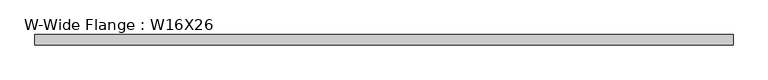
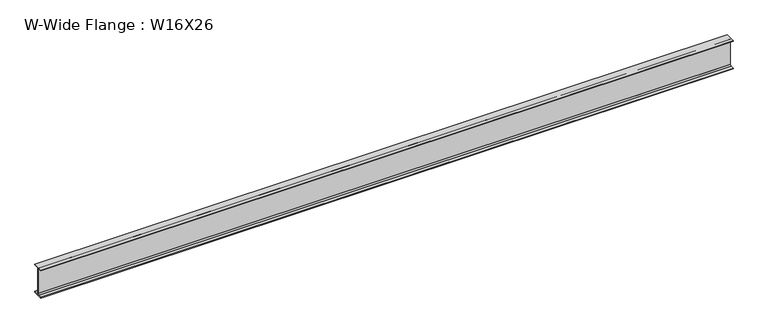
"""IFC4 building model written with IfcOpenShell, lengths in millimetres: beam geometry, W-Wide Flange : W16X26."""

from ifc_helpers import new_model, si_unit, point, frame, frame_2d, origin, place, context, project, spatial, polyline, circle_curve, trimmed, segment, composite_curve, outline, extrude, source, transform, mapped, element, save


def w_wide_flange_w16x26_70125ba5(model_context):
    return source(origin(), model_context, "Body", "SweptSolid", [
        extrude(outline(composite_curve([segment(polyline([(69.85, -190.627), (69.85, -199.39), (-69.85, -199.39), (-69.85, -190.627), (-21.3995, -190.627)]), True, "CONTINUOUS"), segment(trimmed(circle_curve(frame_2d((-21.3995, -172.4025)), 18.2245), [point((-21.3995, -190.627))], [point((-3.175, -172.4025))], True, "CARTESIAN"), True, "CONTINUOUS"), segment(polyline([(-3.175, -172.4025), (-3.175, 172.4025)]), True, "CONTINUOUS"), segment(trimmed(circle_curve(frame_2d((-21.3995, 172.4025)), 18.2245), [point((-3.175, 172.4025))], [point((-21.3995, 190.627))], True, "CARTESIAN"), True, "CONTINUOUS"), segment(polyline([(-21.3995, 190.627), (-69.85, 190.627), (-69.85, 199.39), (69.85, 199.39), (69.85, 190.627), (21.3995, 190.627)]), True, "CONTINUOUS"), segment(trimmed(circle_curve(frame_2d((21.3995, 172.4025)), 18.2245), [point((21.3995, 190.627))], [point((3.175, 172.4025))], True, "CARTESIAN"), True, "CONTINUOUS"), segment(polyline([(3.175, 172.4025), (3.175, -172.4025)]), True, "CONTINUOUS"), segment(trimmed(circle_curve(frame_2d((21.3995, -172.4025)), 18.2245), [point((3.175, -172.4025))], [point((21.3995, -190.627))], True, "CARTESIAN"), True, "CONTINUOUS"), segment(polyline([(21.3995, -190.627), (69.85, -190.627)]), True, "CONTINUOUS")], self_intersect=False)), frame((-4672.838, 0.0, 0.0), z_axis=(1.0, 0.0, 0.0), x_axis=(0.0, 1.0, 0.0)), (0.0, 0.0, 1.0), 9340.088),
    ])


if __name__ == "__main__":
    model = new_model("IFC4")
    model_context = context("Model", 3, world=origin())
    ifc_project = project(units=[si_unit("LENGTHUNIT", "METRE", prefix="MILLI")], contexts=[model_context])
    site = spatial("IfcSite", under=ifc_project)
    building = spatial("IfcBuilding", under=site)
    placement = place(None, origin())
    w_wide_flange_w16x26_shape = w_wide_flange_w16x26_70125ba5(model_context)
    element("IfcBeam", 1, ObjectType="W-Wide Flange : W16X26", at=placement, inside=building, context=model_context, shape_type="MappedRepresentation", body=[
        mapped(w_wide_flange_w16x26_shape, transform((0.0, 0.0, 0.0), x_axis=(1.0, 0.0, 0.0), y_axis=(0.0, 1.0, 0.0), z_axis=(0.0, 0.0, 1.0))),
    ])
    save(model, "model.ifc")

# Revit data of these elements
# Type "W-Wide Flange : W16X26"
#   Assembly Code = "B10"
#   W = 26
#   Length [instance default] = 1524 mm
#   bf = 139.7 mm
#   d = 398.78 mm
#   k = 26.988 mm
#   k2 = 18.225 mm
#   tf = 8.763 mm
#   tw = 6.35 mm
#   A = 0.00495483 m²
#   Structural Material [instance default] = Steel ASTM A992
# Element 1 (IfcBeam, "W-Wide Flange : W16X26")
#   Structural Material = Aluminum, Anodized Red
#   Materials on its faces: "Aluminum, Anodized Red"
# Materials
#   "Steel ASTM A992": class "Metal", colour RGB 128 0 0, transparency 0, Description = "Structural steel 50ksi", Cost = 0
#   "Aluminum, Anodized Red": class "Metal", colour RGB 120 120 120, transparency 0, Description = "Anodized aluminum, red", Cost = 0
